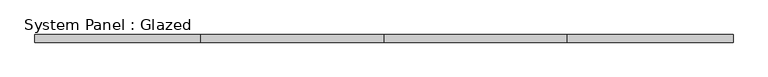
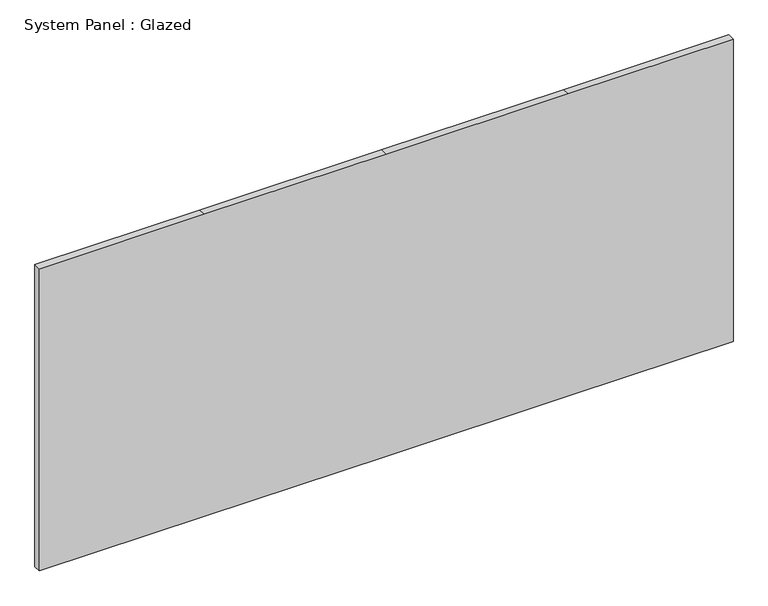
"""IFC4 building model written with IfcOpenShell, lengths in millimetres: plate geometry, System Panel : Glazed."""

from ifc_helpers import new_model, si_unit, frame, origin, place, context, project, spatial, polyline, outline, extrude, source, transform, mapped, element, save


def system_panel_glazed_0cb69296(model_context):
    return source(origin(), model_context, "Body", "SweptSolid", [
        extrude(outline(polyline([(0.0, -2289.0), (0.0, -1200.0), (0.0, 0.0), (0.0, 1200.0), (0.0, 2289.0), (2110.0, 2289.0), (2110.0, 1200.0), (2110.0, 0.0), (2110.0, -1200.0), (2110.0, -2289.0), (0.0, -2289.0)])), frame((0.0, -25.0, 0.0), z_axis=(0.0, 1.0, 0.0), x_axis=(0.0, 0.0, 1.0)), (0.0, 0.0, 1.0), 50.0),
    ])


if __name__ == "__main__":
    model = new_model("IFC4")
    model_context = context("Model", 3, world=origin())
    ifc_project = project(units=[si_unit("LENGTHUNIT", "METRE", prefix="MILLI")], contexts=[model_context])
    site = spatial("IfcSite", under=ifc_project)
    building = spatial("IfcBuilding", under=site)
    placement = place(None, origin())
    system_panel_glazed_shape = system_panel_glazed_0cb69296(model_context)
    element("IfcPlate", 1, ObjectType="System Panel : Glazed", at=placement, inside=building, context=model_context, shape_type="MappedRepresentation", body=[
        mapped(system_panel_glazed_shape, transform((0.0, 0.0, 0.0), x_axis=(1.0, 0.0, 0.0), y_axis=(0.0, 1.0, 0.0), z_axis=(0.0, 0.0, 1.0))),
    ])
    save(model, "model.ifc")

# Revit data of these elements
# Type "System Panel : Glazed"
#   Type Mark = "CW-GLASS"
# Element 1 (IfcPlate, "System Panel : Glazed")
#   Materials on its faces: "Glass_Clear"
# Materials
#   "Glass_Clear": class "Glass", colour RGB 128 128 255, transparency 0.8, Comments = "Rendering appearance not upgraded ", Cost = 0
